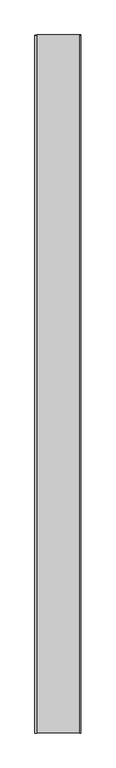
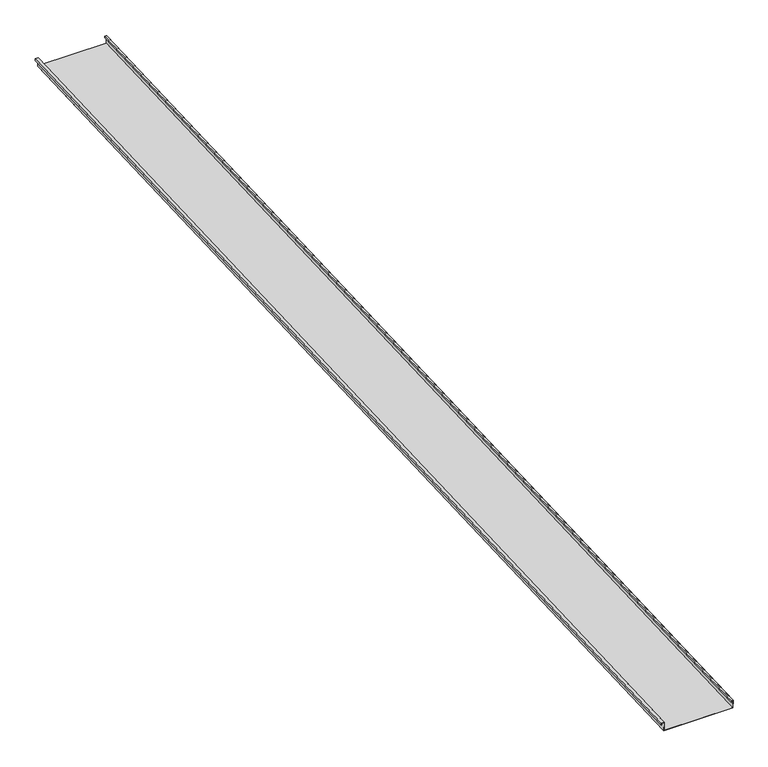
"""IFC4 building model written with IfcOpenShell, lengths in millimetres: proxy geometry, Generic Models 2:Generic Models 2:310765:Generic Models 2:310765 : Generic Models 2:Generic Models 2:310765:118 : Generic Models 2:Generic Models 2:310765:Generic Models 2:310765 : Generic Models 2:Generic Models 2:310765:300385."""

from ifc_helpers import new_model, si_unit, frame, origin, place, context, project, spatial, polyline, outline, extrude, source, transform, mapped, element, save


def generic_models_e10171f5(model_context):
    return source(origin(), model_context, "Body", "SweptSolid", [
        extrude(outline(polyline([(1.5875, 0.0), (1.5875, 50.8), (407.9875, 50.8), (407.9875, 1.5875), (396.875, 1.5875), (396.875, 11.1125), (398.4625, 11.1125), (398.4625, 3.175), (406.4, 3.175), (406.4, 49.2125), (3.175, 49.2125), (3.175, -1.5874999), (-14.2875, -1.5874999), (-14.2875, 9.525), (-12.7, 9.525), (-12.7, 0.0), (1.5875, 0.0)])), frame((665435.1429738, -581354.4345603, 3902.6697972), z_axis=(0.0, 0.9991330730923568, 0.041630544712067834), x_axis=(1.0, 0.0, 0.0)), (0.0, 0.0, 1.0), 6400.8),
    ])


if __name__ == "__main__":
    model = new_model("IFC4")
    model_context = context("Model", 3, world=origin())
    ifc_project = project(units=[si_unit("LENGTHUNIT", "METRE", prefix="MILLI")], contexts=[model_context])
    site = spatial("IfcSite", under=ifc_project)
    building = spatial("IfcBuilding", under=site)
    placement = place(None, origin())
    generic_models_shape = generic_models_e10171f5(model_context)
    element("IfcBuildingElementProxy", 1, Name="Generic Models 2:Generic Models 2:310765:Generic Models 2:310765 : Generic Models 2:Generic Models 2:310765:118 : Generic Models 2:Generic Models 2:310765:Generic Models 2:310765 : Generic Models 2:Generic Models 2:310765:300385", ObjectType="Generic Models 2:Generic Models 2:310765:Generic Models 2:310765 : Generic Models 2:Generic Models 2:310765:118 : Generic Models 2:Generic Models 2:310765:Generic Models 2:310765 : Generic Models 2:Generic Models 2:310765:300385", at=placement, inside=building, context=model_context, shape_type="MappedRepresentation", body=[
        mapped(generic_models_shape, transform((0.0, 0.0, 0.0), x_axis=(1.0, 0.0, 0.0), y_axis=(0.0, 1.0, 0.0), z_axis=(0.0, 0.0, 1.0))),
    ])
    save(model, "model.ifc")

# Revit data of these elements
# Type "Generic Models 2:Generic Models 2:310765:Generic Models 2:310765 : Generic Models 2:Generic Models 2:310765:118 : Generic Models 2:Generic Models 2:310765:Generic Models 2:310765 : Generic Models 2:Generic Models 2:310765:300385"
#   NameOverride = "Generic Models 2:Generic Models 2:310765:Generic Models 2:310765 : Generic Models 2:Generic Models 2:310765:300385"
#   ObjectTypeOverride = "Generic Models 2:310765 : Generic Models 2:Generic Models 2:310765"
#   Reference = "Generic Models 2"
#   Tag = "300385"
# Element 1 (IfcBuildingElementProxy, "Generic Models 2:Generic Models 2:310765:Generic Models 2:310765 : Generic Models 2:Generic Models 2:310765:118 : Generic Models 2:Generic Models 2:310765:Generic Models 2:310765 : Generic Models 2:Generic Models 2:310765:300385")
#   Materials on its faces: "THERMAL BROKEN ALUMINUM STOREFRONT FOR POLYCARBONATE"
# Materials
#   "THERMAL BROKEN ALUMINUM STOREFRONT FOR POLYCARBONATE": class "Unassigned", colour RGB 244 244 244, transparency 0, Keynote = "M07611300.01", Cost = 0
